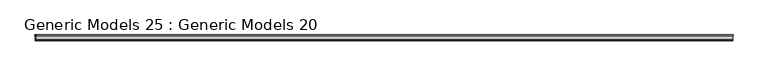
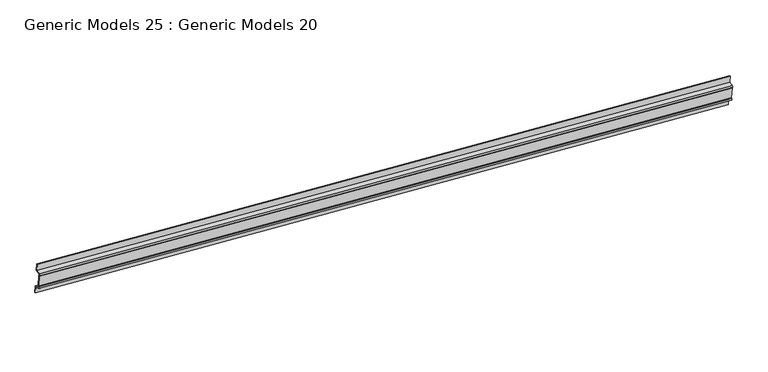
"""IFC4 building model written with IfcOpenShell, lengths in millimetres: proxy geometry, Generic Models 25 : Generic Models 20."""

from ifc_helpers import new_model, si_unit, point, frame, frame_2d, origin, place, context, project, spatial, polyline, circle_curve, trimmed, segment, composite_curve, outline, extrude, source, transform, mapped, element, save


def generic_models_25_generic_models_20_4f4f0fa0(model_context):
    return source(origin(), model_context, "Body", "SweptSolid", [
        extrude(outline(composite_curve([segment(polyline([(-1.5875, -49.974669), (-10.8316343, -47.9357718)]), True, "CONTINUOUS"), segment(trimmed(circle_curve(frame_2d((-10.31875, -45.6104113)), 2.38125), [point((-10.8316343, -47.9357718))], [point((-11.90625, -43.8355324))], False, "CARTESIAN"), True, "CONTINUOUS"), segment(trimmed(circle_curve(frame_2d((-13.49375, -42.0606534)), 2.38125), [point((-11.90625, -43.8355324))], [point((-11.1125, -42.0606534))], True, "CARTESIAN"), True, "CONTINUOUS"), segment(polyline([(-11.1125, -42.0606534), (-11.1125, -21.4393465)]), True, "CONTINUOUS"), segment(trimmed(circle_curve(frame_2d((-13.49375, -21.4393465)), 2.38125), [point((-11.1125, -21.4393465))], [point((-11.90625, -19.6644676))], True, "CARTESIAN"), True, "CONTINUOUS"), segment(trimmed(circle_curve(frame_2d((-10.31875, -17.8895886)), 2.38125), [point((-11.90625, -19.6644676))], [point((-10.8316343, -15.5642282))], False, "CARTESIAN"), True, "CONTINUOUS"), segment(polyline([(-10.8316343, -15.5642282), (-1.5875, -13.525331), (-1.5875, 0.0), (0.0, 0.0), (0.0, -14.8008452), (-10.4897114, -17.1144684)]), True, "CONTINUOUS"), segment(trimmed(circle_curve(frame_2d((-10.31875, -17.8895886)), 0.79375), [point((-10.4897114, -17.1144684))], [point((-10.8479167, -18.4812149))], True, "CARTESIAN"), True, "CONTINUOUS"), segment(trimmed(circle_curve(frame_2d((-13.49375, -21.4393465)), 3.96875), [point((-10.8479167, -18.4812149))], [point((-9.525, -21.4393465))], False, "CARTESIAN"), True, "CONTINUOUS"), segment(polyline([(-9.525, -21.4393465), (-9.525, -42.0606534)]), True, "CONTINUOUS"), segment(trimmed(circle_curve(frame_2d((-13.49375, -42.0606534)), 3.96875), [point((-9.525, -42.0606534))], [point((-10.8479167, -45.0187851))], False, "CARTESIAN"), True, "CONTINUOUS"), segment(trimmed(circle_curve(frame_2d((-10.31875, -45.6104113)), 0.79375), [point((-10.8479167, -45.0187851))], [point((-10.4897114, -46.3855315))], True, "CARTESIAN"), True, "CONTINUOUS"), segment(polyline([(-10.4897114, -46.3855315), (0.0, -48.6991547), (0.0, -63.4999999), (-1.5875, -63.4999999), (-1.5875, -49.974669)]), True, "CONTINUOUS")], self_intersect=False)), frame((28940.214405, 25522.8906612, 272602.0634595), z_axis=(-0.9980525759468354, 0.0, 0.06237832673201837), x_axis=(0.0, 1.0, 0.0)), (0.0, 0.0, 1.0), 1498.6),
    ])


if __name__ == "__main__":
    model = new_model("IFC4")
    model_context = context("Model", 3, world=origin())
    ifc_project = project(units=[si_unit("LENGTHUNIT", "METRE", prefix="MILLI")], contexts=[model_context])
    site = spatial("IfcSite", under=ifc_project)
    building = spatial("IfcBuilding", under=site)
    placement = place(None, origin())
    generic_models_25_generic_models_20_shape = generic_models_25_generic_models_20_4f4f0fa0(model_context)
    element("IfcBuildingElementProxy", 1, Name="Generic Models 25 : Generic Models 20", ObjectType="Generic Models 25 : Generic Models 20", at=placement, inside=building, context=model_context, shape_type="MappedRepresentation", body=[
        mapped(generic_models_25_generic_models_20_shape, transform((0.0, 0.0, 0.0), x_axis=(1.0, 0.0, 0.0), y_axis=(0.0, 1.0, 0.0), z_axis=(0.0, 0.0, 1.0))),
    ])
    save(model, "model.ifc")

# Revit data of these elements
# Element 1 (IfcBuildingElementProxy, "Generic Models 25 : Generic Models 20")
#   Materials on its faces: "1/2\" DEEP GALV. HORTZ. HAT CHANNEL @ XX O.C."
# Materials
#   "1/2\" DEEP GALV. HORTZ. HAT CHANNEL @ XX O.C.": class "Generic", colour RGB 212 212 212, transparency 0, Cost = 0
